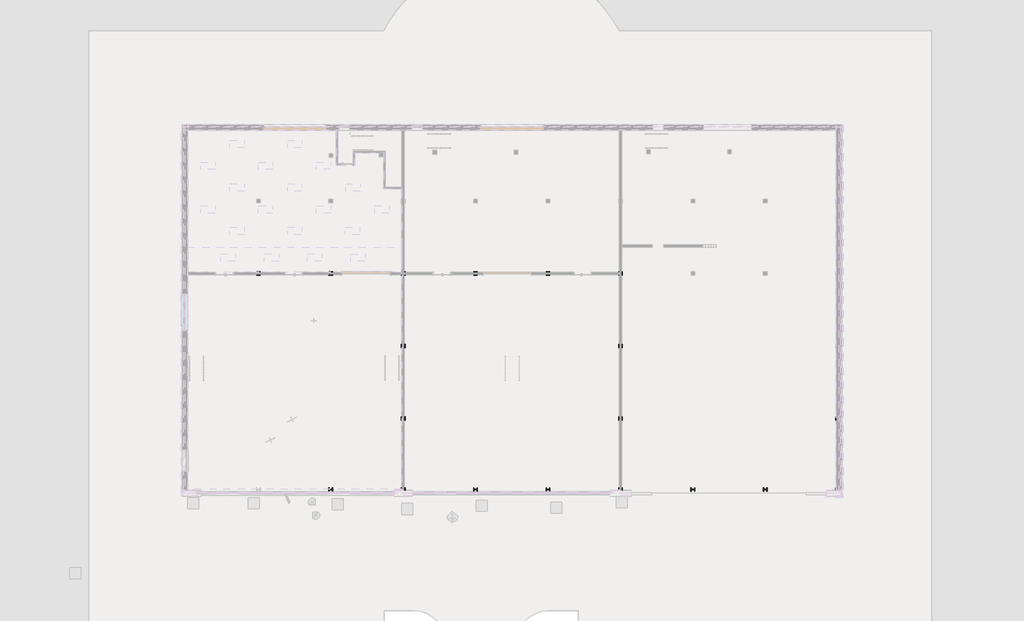
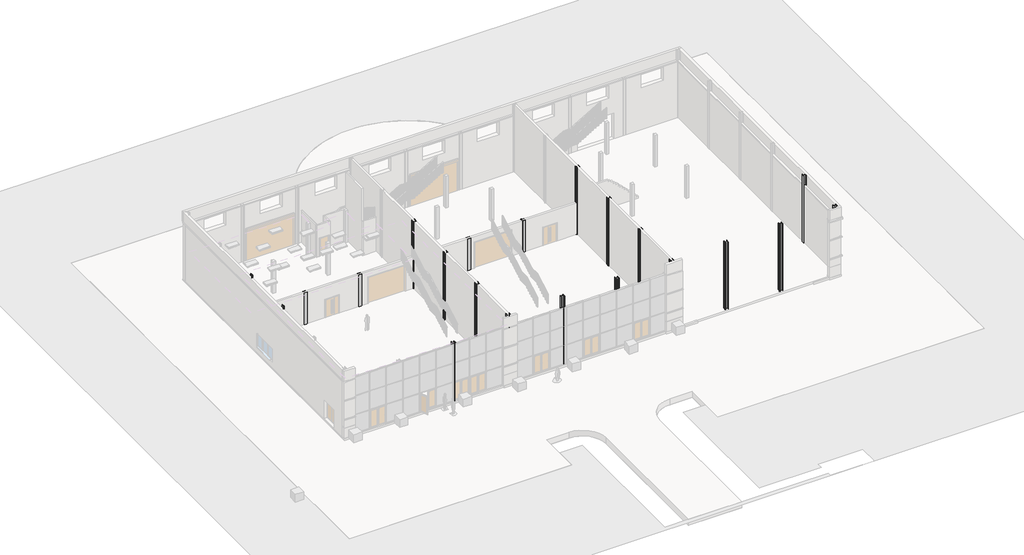
# One storey, part 5 of 13: 21 columns, 21 slabs, 8 footings.
"""IFC4 building model written with IfcOpenShell, lengths in millimetres."""

import ifcopenshell
import ifcopenshell.guid

model = None  # the IFC model being written
_history = None  # IfcOwnerHistory: only IFC2X3 demands one
_inside = {}  # id of a spatial element -> (the spatial element, [elements in it])
_under = {}  # id of a project, library or spatial element -> (it, [spatial elements below it])
_declared = {}  # id of a project -> (the project, [libraries it declares])
_typed = {}  # id of a type object -> (the type object, [elements of that type])
_made_of = {}  # id of a material, layer set ... -> (it, [elements and type objects made of it])


def new_model(schema):
    """Start an empty IFC model of exactly this schema.

    Asked for "IFC4X3", IfcOpenShell would pick the latest addendum, in which some entities
    have other attributes; the version numbers below select the first issue.
    IFC2X3 requires an IfcOwnerHistory on every rooted entity: one is made here for all.
    """
    global model, _history
    if schema == "IFC4X3":
        model = ifcopenshell.file(schema_version=(4, 3, 0, 0))
    else:
        model = ifcopenshell.file(schema=schema)
    _inside.clear()
    _under.clear()
    _declared.clear()
    _typed.clear()
    _made_of.clear()
    _history = None
    if model.schema == "IFC2X3":
        org = make("IfcOrganization", Name="unknown")
        user = make(
            "IfcPersonAndOrganization",
            ThePerson=make("IfcPerson", FamilyName="unknown"),
            TheOrganization=org,
        )
        app = make(
            "IfcApplication",
            ApplicationDeveloper=org,
            Version="unknown",
            ApplicationFullName="unknown",
            ApplicationIdentifier="unknown",
        )
        _history = make(
            "IfcOwnerHistory",
            OwningUser=user,
            OwningApplication=app,
            ChangeAction="ADDED",
            CreationDate=0,
        )
    return model


def make(cls, **values):
    """One entity of the class cls with the attributes given. An attribute that is None is left unset."""
    return model.create_entity(
        cls, **{name: value for name, value in values.items() if value is not None}
    )


def rooted(cls, **values):
    """An entity with a GlobalId (a new one), such as an element, a storey or a relation."""
    return make(cls, GlobalId=ifcopenshell.guid.new(), OwnerHistory=_history, **values)


def si_unit(unit_type, name, prefix=None):
    """IfcSIUnit, for example si_unit("LENGTHUNIT", "METRE", prefix="MILLI")."""
    return make("IfcSIUnit", UnitType=unit_type, Prefix=prefix, Name=name)


def assignment(units):
    """IfcUnitAssignment: the units of a project."""
    return None if units is None else make("IfcUnitAssignment", Units=units)


def point(xyz):
    """IfcCartesianPoint."""
    return None if xyz is None else make("IfcCartesianPoint", Coordinates=xyz)


def direction(xyz):
    """IfcDirection."""
    return None if xyz is None else make("IfcDirection", DirectionRatios=xyz)


def frame(location, z_axis=None, x_axis=None):
    """IfcAxis2Placement3D, a coordinate frame: its origin and axes. An axis left out is left unset."""
    return make(
        "IfcAxis2Placement3D",
        Location=point(location),
        Axis=direction(z_axis),
        RefDirection=direction(x_axis),
    )


def frame_2d(location, x_axis=None):
    """IfcAxis2Placement2D, a coordinate frame in the plane: its origin and x axis."""
    return make(
        "IfcAxis2Placement2D", Location=point(location), RefDirection=direction(x_axis)
    )


def origin():
    """The frame at (0, 0, 0) with its axes left unset."""
    return frame((0.0, 0.0, 0.0))


def place(relative_to, where):
    """IfcLocalPlacement: puts the frame where relative to a parent placement (None: the world)."""
    return make(
        "IfcLocalPlacement", PlacementRelTo=relative_to, RelativePlacement=where
    )


def context(
    kind, dimensions, precision=None, world=None, true_north=None, identifier=None
):
    """IfcGeometricRepresentationContext, for example the 3D "Model" context."""
    return make(
        "IfcGeometricRepresentationContext",
        ContextIdentifier=identifier,
        ContextType=kind,
        CoordinateSpaceDimension=dimensions,
        Precision=precision,
        WorldCoordinateSystem=world,
        TrueNorth=true_north,
    )


def project(units=None, contexts=None):
    """IfcProject with its units and contexts."""
    return rooted(
        "IfcProject",
        Name="project",
        RepresentationContexts=contexts,
        UnitsInContext=assignment(units),
    )


def spatial(cls, under=None, at=None, **own):
    """A site, building, storey or space (cls), placed at a placement, below another one or the project."""
    s = rooted(cls, ObjectPlacement=at, **own)
    if under is not None:
        _under.setdefault(under.id(), (under, []))[1].append(s)
    return s


def polyline(points):
    """IfcPolyline through the points."""
    return make("IfcPolyline", Points=[point(p) for p in points])


def circle_curve(where, radius):
    """IfcCircle in the frame where."""
    return make("IfcCircle", Position=where, Radius=radius)


def trimmed(basis, trim1, trim2, sense, master):
    """IfcTrimmedCurve: the piece of a basis curve between two trims."""
    return make(
        "IfcTrimmedCurve",
        BasisCurve=basis,
        Trim1=trim1,
        Trim2=trim2,
        SenseAgreement=sense,
        MasterRepresentation=master,
    )


def segment(curve, same_sense, transition):
    """IfcCompositeCurveSegment."""
    return make(
        "IfcCompositeCurveSegment",
        Transition=transition,
        SameSense=same_sense,
        ParentCurve=curve,
    )


def composite_curve(segments, self_intersect=None):
    """IfcCompositeCurve: segments joined end to end."""
    return make("IfcCompositeCurve", Segments=segments, SelfIntersect=self_intersect)


def outline(outer, holes=None, kind="AREA"):
    """IfcArbitraryClosedProfileDef: a profile drawn as a closed curve; with holes, ...WithVoids."""
    if holes is None:
        return make("IfcArbitraryClosedProfileDef", ProfileType=kind, OuterCurve=outer)
    return make(
        "IfcArbitraryProfileDefWithVoids",
        ProfileType=kind,
        OuterCurve=outer,
        InnerCurves=holes,
    )


def extrude(swept, where, along, depth):
    """IfcExtrudedAreaSolid: the profile swept, set in the frame where, extruded along a direction by depth."""
    return make(
        "IfcExtrudedAreaSolid",
        SweptArea=swept,
        Position=where,
        ExtrudedDirection=direction(along),
        Depth=depth,
    )


def faces_of(points, faces, orient=None, outer=None):
    """IfcFace entities. A face is a list of loops; a loop is a list of indices into points, from 0.

    orient and outer hold one flag for each loop. By default every Orientation is true, the
    first loop of a face is its IfcFaceOuterBound and the others are IfcFaceBound.
    """
    made = []
    for i, loops in enumerate(faces):
        bounds = []
        for j, loop in enumerate(loops):
            is_outer = j == 0 if outer is None else outer[i][j]
            bounds.append(
                make(
                    "IfcFaceOuterBound" if is_outer else "IfcFaceBound",
                    Bound=make("IfcPolyLoop", Polygon=[points[k] for k in loop]),
                    Orientation=True if orient is None else orient[i][j],
                )
            )
        made.append(make("IfcFace", Bounds=bounds))
    return made


def faceted_brep(points, faces, orient=None, outer=None, voids=None):
    """IfcFacetedBrep: a solid bounded by flat faces; with voids (closed shells), ...WithVoids."""
    shared = [point(p) for p in points]
    hull = make("IfcClosedShell", CfsFaces=faces_of(shared, faces, orient, outer))
    if voids is None:
        return make("IfcFacetedBrep", Outer=hull)
    return make(
        "IfcFacetedBrepWithVoids",
        Outer=hull,
        Voids=[
            make(cls, CfsFaces=faces_of(shared, fs, o, b)) for cls, fs, o, b in voids
        ],
    )


def shape(context_of_items, identifier, shape_type, items):
    """IfcShapeRepresentation: the items that make up one representation, for example the "Body"."""
    return make(
        "IfcShapeRepresentation",
        ContextOfItems=context_of_items,
        RepresentationIdentifier=identifier,
        RepresentationType=shape_type,
        Items=items,
    )


def source(mapping_origin, context_of_items, identifier, shape_type, items):
    """IfcRepresentationMap: a shape defined once, which mapped items show again and again."""
    return make(
        "IfcRepresentationMap",
        MappingOrigin=mapping_origin,
        MappedRepresentation=shape(context_of_items, identifier, shape_type, items),
    )


def transform(
    local_origin,
    x_axis=None,
    y_axis=None,
    z_axis=None,
    scale=None,
    scale2=None,
    scale3=None,
    uniform=True,
):
    """IfcCartesianTransformationOperator3D, or its non-uniform kind. x_axis, y_axis, z_axis: its Axis1, 2, 3."""
    if uniform:
        return make(
            "IfcCartesianTransformationOperator3D",
            Axis1=direction(x_axis),
            Axis2=direction(y_axis),
            LocalOrigin=point(local_origin),
            Scale=scale,
            Axis3=direction(z_axis),
        )
    return make(
        "IfcCartesianTransformationOperator3DnonUniform",
        Axis1=direction(x_axis),
        Axis2=direction(y_axis),
        LocalOrigin=point(local_origin),
        Scale=scale,
        Axis3=direction(z_axis),
        Scale2=scale2,
        Scale3=scale3,
    )


def mapped(mapping_source, mapping_target):
    """IfcMappedItem: shows the shape of a source again, moved by a transform."""
    return make(
        "IfcMappedItem", MappingSource=mapping_source, MappingTarget=mapping_target
    )


def made_of(thing, what):
    """Note that an element or type object is made of a material, layer set ...; save() writes the relation."""
    if what is not None:
        _made_of.setdefault(what.id(), (what, []))[1].append(thing)
    return thing


def element(
    cls,
    number,
    at=None,
    inside=None,
    cuts=None,
    type_object=None,
    material=None,
    context=None,
    identifier="Body",
    shape_type=None,
    held_by="IfcProductDefinitionShape",
    body=None,
    shapes=None,
    **own,
):
    """One element of the class cls, such as IfcWall. Its Tag is "e" and its number.

    at: its placement. inside: the storey or other place that contains it. cuts: it is an
    opening in that element (IfcRelVoidsElement). A single representation is given by context,
    identifier, shape_type and body (its items); several are given by shapes. held_by: the class
    of the entity that holds the representations. save() writes the other relations.
    """
    e = rooted(cls, Tag="e%d" % number, ObjectPlacement=at, **own)
    if body is not None:
        shapes = [shape(context, identifier, shape_type, body)]
    if shapes is not None:
        e.Representation = make(held_by, Representations=shapes)
    if inside is not None:
        _inside.setdefault(inside.id(), (inside, []))[1].append(e)
    if cuts is not None:
        rooted(
            "IfcRelVoidsElement", RelatingBuildingElement=cuts, RelatedOpeningElement=e
        )
    if type_object is not None:
        _typed.setdefault(type_object.id(), (type_object, []))[1].append(e)
    return made_of(e, material)


def aggregate(whole, parts):
    """IfcRelAggregates: a whole, such as a stair, and the parts it consists of."""
    return rooted("IfcRelAggregates", RelatingObject=whole, RelatedObjects=parts)


def save(model, path):
    """Write the relations noted so far, then the file.

    IfcRelAggregates (storeys below a building ...), IfcRelContainedInSpatialStructure (elements
    in a storey), IfcRelDefinesByType, IfcRelAssociatesMaterial and IfcRelDeclares: one each for
    every whole, place, type object, material and project.
    """
    for whole, parts in _under.values():
        aggregate(whole, parts)
    for where, things in _inside.values():
        rooted(
            "IfcRelContainedInSpatialStructure",
            RelatedElements=things,
            RelatingStructure=where,
        )
    for kind, things in _typed.values():
        rooted("IfcRelDefinesByType", RelatedObjects=things, RelatingType=kind)
    for what, things in _made_of.values():
        rooted("IfcRelAssociatesMaterial", RelatedObjects=things, RelatingMaterial=what)
    for by, libraries in _declared.values():
        rooted("IfcRelDeclares", RelatingContext=by, RelatedDefinitions=libraries)
    model.write(path)


def uc_universal_column_column_305x305x97uc_f4bfb62a(model_context):
    return source(origin(), model_context, "Body", "SweptSolid", [
        extrude(outline(composite_curve([segment(polyline([(152.65, 153.95), (152.65, 138.55), (20.15, 138.55)]), True, "CONTINUOUS"), segment(trimmed(circle_curve(frame_2d((20.15, 123.35)), 15.2), [point((20.15, 138.55))], [point((4.95, 123.35))], True, "CARTESIAN"), True, "CONTINUOUS"), segment(polyline([(4.95, 123.35), (4.95, -123.35)]), True, "CONTINUOUS"), segment(trimmed(circle_curve(frame_2d((20.15, -123.35)), 15.2), [point((4.95, -123.35))], [point((20.15, -138.55))], True, "CARTESIAN"), True, "CONTINUOUS"), segment(polyline([(20.15, -138.55), (152.65, -138.55), (152.65, -153.95), (-152.65, -153.95), (-152.65, -138.55), (-20.15, -138.55)]), True, "CONTINUOUS"), segment(trimmed(circle_curve(frame_2d((-20.15, -123.35)), 15.2), [point((-20.15, -138.55))], [point((-4.95, -123.35))], True, "CARTESIAN"), True, "CONTINUOUS"), segment(polyline([(-4.95, -123.35), (-4.95, 123.35)]), True, "CONTINUOUS"), segment(trimmed(circle_curve(frame_2d((-20.15, 123.35)), 15.2), [point((-4.95, 123.35))], [point((-20.15, 138.55))], True, "CARTESIAN"), True, "CONTINUOUS"), segment(polyline([(-20.15, 138.55), (-152.65, 138.55), (-152.65, 153.95), (152.65, 153.95)]), True, "CONTINUOUS")], self_intersect=False)), frame((0.0, 0.0, -1500.0), z_axis=(0.0, 0.0, 1.0), x_axis=(1.0, 0.0, 0.0)), (0.0, 0.0, 1.0), 9300.0),
    ])


def uc_universal_column_column_305x305x97uc_8da79b43(model_context):
    return source(origin(), model_context, "Body", "SweptSolid", [
        extrude(outline(composite_curve([segment(polyline([(152.65, -153.95), (-152.65, -153.95), (-152.65, -138.55), (-20.15, -138.55)]), True, "CONTINUOUS"), segment(trimmed(circle_curve(frame_2d((-20.15, -123.35)), 15.2), [point((-20.15, -138.55))], [point((-4.95, -123.35))], True, "CARTESIAN"), True, "CONTINUOUS"), segment(polyline([(-4.95, -123.35), (-4.95, 123.35)]), True, "CONTINUOUS"), segment(trimmed(circle_curve(frame_2d((-20.15, 123.35)), 15.2), [point((-4.95, 123.35))], [point((-20.15, 138.55))], True, "CARTESIAN"), True, "CONTINUOUS"), segment(polyline([(-20.15, 138.55), (-152.65, 138.55), (-152.65, 153.95), (152.65, 153.95), (152.65, 138.55), (20.15, 138.55)]), True, "CONTINUOUS"), segment(trimmed(circle_curve(frame_2d((20.15, 123.35)), 15.2), [point((20.15, 138.55))], [point((4.95, 123.35))], True, "CARTESIAN"), True, "CONTINUOUS"), segment(polyline([(4.95, 123.35), (4.95, -123.35)]), True, "CONTINUOUS"), segment(trimmed(circle_curve(frame_2d((20.15, -123.35)), 15.2), [point((4.95, -123.35))], [point((20.15, -138.55))], True, "CARTESIAN"), True, "CONTINUOUS"), segment(polyline([(20.15, -138.55), (152.65, -138.55), (152.65, -153.95)]), True, "CONTINUOUS")], self_intersect=False)), frame((0.0, 0.0, -1500.0), z_axis=(0.0, 0.0, 1.0), x_axis=(1.0, 0.0, 0.0)), (0.0, 0.0, 1.0), 9300.0),
    ])


def uc_universal_column_column_305x305x97uc_43a052ce(model_context):
    return source(origin(), model_context, "Body", "SweptSolid", [
        extrude(outline(composite_curve([segment(polyline([(152.65, 153.95), (152.65, 138.55), (20.15, 138.55)]), True, "CONTINUOUS"), segment(trimmed(circle_curve(frame_2d((20.15, 123.35)), 15.2), [point((20.15, 138.55))], [point((4.95, 123.35))], True, "CARTESIAN"), True, "CONTINUOUS"), segment(polyline([(4.95, 123.35), (4.95, -123.35)]), True, "CONTINUOUS"), segment(trimmed(circle_curve(frame_2d((20.15, -123.35)), 15.2), [point((4.95, -123.35))], [point((20.15, -138.55))], True, "CARTESIAN"), True, "CONTINUOUS"), segment(polyline([(20.15, -138.55), (152.65, -138.55), (152.65, -153.95), (-152.65, -153.95), (-152.65, -138.55), (-20.15, -138.55)]), True, "CONTINUOUS"), segment(trimmed(circle_curve(frame_2d((-20.15, -123.35)), 15.2), [point((-20.15, -138.55))], [point((-4.95, -123.35))], True, "CARTESIAN"), True, "CONTINUOUS"), segment(polyline([(-4.95, -123.35), (-4.95, 123.35)]), True, "CONTINUOUS"), segment(trimmed(circle_curve(frame_2d((-20.15, 123.35)), 15.2), [point((-4.95, 123.35))], [point((-20.15, 138.55))], True, "CARTESIAN"), True, "CONTINUOUS"), segment(polyline([(-20.15, 138.55), (-152.65, 138.55), (-152.65, 153.95), (152.65, 153.95)]), True, "CONTINUOUS")], self_intersect=False)), frame((0.0, 0.0, -1500.0), z_axis=(0.0, 0.0, 1.0), x_axis=(1.0, 0.0, 0.0)), (0.0, 0.0, 1.0), 8100.0),
    ])


def pad_foundation_rectangular_1000x1000x500_ed6229e9(model_context):
    return source(origin(), model_context, "Body", "SweptSolid", [
        extrude(outline(polyline([(500.0, 500.0), (500.0, -500.0), (-500.0, -500.0), (-500.0, 500.0), (500.0, 500.0)])), frame((0.0, 0.0, -500.0), z_axis=(0.0, 0.0, 1.0), x_axis=(1.0, 0.0, 0.0)), (0.0, 0.0, 1.0), 500.0),
    ])


model = new_model("IFC4")

# Units and contexts
model_context = context("Model", 3, world=origin())
ifc_project = project(units=[si_unit("LENGTHUNIT", "METRE", prefix="MILLI")], contexts=[model_context])

# Site, building, storey
site = spatial("IfcSite", under=ifc_project)
building = spatial("IfcBuilding", under=site)
storey = spatial("IfcBuildingStorey", under=building, Name="L0 - Ground Floor (Shadows On)", Elevation=0.0)

# Columns
placement = place(None, origin())
element("IfcColumn", 1, ObjectType="Concrete Square : 300 x 300mm", at=placement, inside=storey, context=model_context, shape_type="SweptSolid", body=[
    extrude(outline(polyline([(-989.5553457, -5208.7619082), (-1289.5553457, -5208.7619082), (-1289.5553457, -4908.7619082), (-989.5553457, -4908.7619082), (-989.5553457, -5208.7619082)])), frame((0.0, 0.0, -1500.0), z_axis=(0.0, 0.0, 1.0), x_axis=(1.0, 0.0, 0.0)), (0.0, 0.0, 1.0), 5200.0),
])
element("IfcColumn", 2, ObjectType="Concrete Square : 300 x 300mm", at=placement, inside=storey, context=model_context, shape_type="SweptSolid", body=[
    extrude(outline(polyline([(5010.4446543, -5208.7619082), (4710.4446543, -5208.7619082), (4710.4446543, -4908.7619082), (5010.4446543, -4908.7619082), (5010.4446543, -5208.7619082)])), frame((0.0, 0.0, -1500.0), z_axis=(0.0, 0.0, 1.0), x_axis=(1.0, 0.0, 0.0)), (0.0, 0.0, 1.0), 5200.0),
])
element("IfcColumn", 3, ObjectType="Concrete Square : 300 x 300mm", at=placement, inside=storey, context=model_context, shape_type="SweptSolid", body=[
    extrude(outline(polyline([(17010.4446543, -5208.7619082), (16710.4446543, -5208.7619082), (16710.4446543, -4908.7619082), (17010.4446543, -4908.7619082), (17010.4446543, -5208.7619082)])), frame((0.0, 0.0, -1500.0), z_axis=(0.0, 0.0, 1.0), x_axis=(1.0, 0.0, 0.0)), (0.0, 0.0, 1.0), 5200.0),
])
element("IfcColumn", 4, ObjectType="Concrete Square : 300 x 300mm", at=placement, inside=storey, context=model_context, shape_type="SweptSolid", body=[
    extrude(outline(polyline([(23010.4446543, -5208.7619082), (22710.4446543, -5208.7619082), (22710.4446543, -4908.7619082), (23010.4446543, -4908.7619082), (23010.4446543, -5208.7619082)])), frame((0.0, 0.0, -1500.0), z_axis=(0.0, 0.0, 1.0), x_axis=(1.0, 0.0, 0.0)), (0.0, 0.0, 1.0), 5200.0),
])
element("IfcColumn", 5, ObjectType="UC-Universal Column-Column : 305x305x97UC", at=placement, inside=storey, context=model_context, shape_type="SweptSolid", body=[
    extrude(outline(composite_curve([segment(polyline([(-7293.5053457, -10906.1119082), (-7278.1053457, -10906.1119082), (-7278.1053457, -11038.6119082)]), True, "CONTINUOUS"), segment(trimmed(circle_curve(frame_2d((-7262.9053457, -11038.6119082)), 15.2), [point((-7278.1053457, -11038.6119082))], [point((-7262.9053457, -11053.8119082))], True, "CARTESIAN"), True, "CONTINUOUS"), segment(polyline([(-7262.9053457, -11053.8119082), (-7016.2053457, -11053.8119082)]), True, "CONTINUOUS"), segment(trimmed(circle_curve(frame_2d((-7016.2053457, -11038.6119082)), 15.2), [point((-7016.2053457, -11053.8119082))], [point((-7001.0053457, -11038.6119082))], True, "CARTESIAN"), True, "CONTINUOUS"), segment(polyline([(-7001.0053457, -11038.6119082), (-7001.0053457, -10906.1119082), (-6985.6053457, -10906.1119082), (-6985.6053457, -11211.4119082), (-7001.0053457, -11211.4119082), (-7001.0053457, -11078.9119082)]), True, "CONTINUOUS"), segment(trimmed(circle_curve(frame_2d((-7016.2053457, -11078.9119082)), 15.2), [point((-7001.0053457, -11078.9119082))], [point((-7016.2053457, -11063.7119082))], True, "CARTESIAN"), True, "CONTINUOUS"), segment(polyline([(-7016.2053457, -11063.7119082), (-7262.9053457, -11063.7119082)]), True, "CONTINUOUS"), segment(trimmed(circle_curve(frame_2d((-7262.9053457, -11078.9119082)), 15.2), [point((-7262.9053457, -11063.7119082))], [point((-7278.1053457, -11078.9119082))], True, "CARTESIAN"), True, "CONTINUOUS"), segment(polyline([(-7278.1053457, -11078.9119082), (-7278.1053457, -11211.4119082), (-7293.5053457, -11211.4119082), (-7293.5053457, -10906.1119082)]), True, "CONTINUOUS")], self_intersect=False)), frame((0.0, 0.0, -1500.0), z_axis=(0.0, 0.0, 1.0), x_axis=(1.0, 0.0, 0.0)), (0.0, 0.0, 1.0), 9300.0),
])
element("IfcColumn", 6, ObjectType="UC-Universal Column-Column : 305x305x97UC", at=placement, inside=storey, context=model_context, shape_type="SweptSolid", body=[
    extrude(outline(composite_curve([segment(polyline([(-7293.5053457, -4906.1119082), (-7278.1053457, -4906.1119082), (-7278.1053457, -5038.6119082)]), True, "CONTINUOUS"), segment(trimmed(circle_curve(frame_2d((-7262.9053457, -5038.6119082)), 15.2), [point((-7278.1053457, -5038.6119082))], [point((-7262.9053457, -5053.8119082))], True, "CARTESIAN"), True, "CONTINUOUS"), segment(polyline([(-7262.9053457, -5053.8119082), (-7016.2053457, -5053.8119082)]), True, "CONTINUOUS"), segment(trimmed(circle_curve(frame_2d((-7016.2053457, -5038.6119082)), 15.2), [point((-7016.2053457, -5053.8119082))], [point((-7001.0053457, -5038.6119082))], True, "CARTESIAN"), True, "CONTINUOUS"), segment(polyline([(-7001.0053457, -5038.6119082), (-7001.0053457, -4906.1119082), (-6985.6053457, -4906.1119082), (-6985.6053457, -5211.4119082), (-7001.0053457, -5211.4119082), (-7001.0053457, -5078.9119082)]), True, "CONTINUOUS"), segment(trimmed(circle_curve(frame_2d((-7016.2053457, -5078.9119082)), 15.2), [point((-7001.0053457, -5078.9119082))], [point((-7016.2053457, -5063.7119082))], True, "CARTESIAN"), True, "CONTINUOUS"), segment(polyline([(-7016.2053457, -5063.7119082), (-7262.9053457, -5063.7119082)]), True, "CONTINUOUS"), segment(trimmed(circle_curve(frame_2d((-7262.9053457, -5078.9119082)), 15.2), [point((-7262.9053457, -5063.7119082))], [point((-7278.1053457, -5078.9119082))], True, "CARTESIAN"), True, "CONTINUOUS"), segment(polyline([(-7278.1053457, -5078.9119082), (-7278.1053457, -5211.4119082), (-7293.5053457, -5211.4119082), (-7293.5053457, -4906.1119082)]), True, "CONTINUOUS")], self_intersect=False)), frame((0.0, 0.0, -1500.0), z_axis=(0.0, 0.0, 1.0), x_axis=(1.0, 0.0, 0.0)), (0.0, 0.0, 1.0), 9300.0),
])
uc_universal_column_column_305x305x97uc_shape = uc_universal_column_column_305x305x97uc_f4bfb62a(model_context)
element("IfcColumn", 7, ObjectType="UC-Universal Column-Column : 305x305x97UC", at=placement, inside=storey, context=model_context, shape_type="MappedRepresentation", body=[
    mapped(uc_universal_column_column_305x305x97uc_shape, transform((10860.4446543, -17058.7619082, 0.0), x_axis=(0.0, 1.0, 0.0), y_axis=(-1.0, 0.0, 0.0), z_axis=(0.0, 0.0, 1.0))),
])
element("IfcColumn", 8, ObjectType="UC-Universal Column-Column : 305x305x97UC", at=placement, inside=storey, context=model_context, shape_type="MappedRepresentation", body=[
    mapped(uc_universal_column_column_305x305x97uc_shape, transform((28860.4446543, -17058.7619082, 0.0), x_axis=(0.0, 1.0, 0.0), y_axis=(-1.0, 0.0, 0.0), z_axis=(0.0, 0.0, 1.0))),
])
element("IfcColumn", 9, ObjectType="UC-Universal Column-Column : 305x305x97UC", at=placement, inside=storey, context=model_context, shape_type="MappedRepresentation", body=[
    mapped(uc_universal_column_column_305x305x97uc_shape, transform((10860.4446543, -11058.7619082, 0.0), x_axis=(0.0, 1.0, 0.0), y_axis=(-1.0, 0.0, 0.0), z_axis=(0.0, 0.0, 1.0))),
])
element("IfcColumn", 10, ObjectType="UC-Universal Column-Column : 305x305x97UC", at=placement, inside=storey, context=model_context, shape_type="MappedRepresentation", body=[
    mapped(uc_universal_column_column_305x305x97uc_shape, transform((28860.4446543, -11058.7619082, 0.0), x_axis=(0.0, 1.0, 0.0), y_axis=(-1.0, 0.0, 0.0), z_axis=(0.0, 0.0, 1.0))),
])
element("IfcColumn", 11, ObjectType="UC-Universal Column-Column : 305x305x97UC", at=placement, inside=storey, context=model_context, shape_type="MappedRepresentation", body=[
    mapped(uc_universal_column_column_305x305x97uc_shape, transform((10860.4446543, -5058.7619082, 0.0), x_axis=(0.0, 1.0, 0.0), y_axis=(-1.0, 0.0, 0.0), z_axis=(0.0, 0.0, 1.0))),
])
element("IfcColumn", 12, ObjectType="UC-Universal Column-Column : 305x305x97UC", at=placement, inside=storey, context=model_context, shape_type="MappedRepresentation", body=[
    mapped(uc_universal_column_column_305x305x97uc_shape, transform((28860.4446543, -5058.7619082, 0.0), x_axis=(0.0, 1.0, 0.0), y_axis=(-1.0, 0.0, 0.0), z_axis=(0.0, 0.0, 1.0))),
])
element("IfcColumn", 13, ObjectType="UC-Universal Column-Column : 305x305x97UC", at=placement, inside=storey, context=model_context, shape_type="MappedRepresentation", body=[
    mapped(uc_universal_column_column_305x305x97uc_shape, transform((10860.4446543, -22948.7619082, 0.0), x_axis=(0.0, 1.0, 0.0), y_axis=(-1.0, 0.0, 0.0), z_axis=(0.0, 0.0, 1.0))),
])
element("IfcColumn", 14, ObjectType="UC-Universal Column-Column : 305x305x97UC", at=placement, inside=storey, context=model_context, shape_type="MappedRepresentation", body=[
    mapped(uc_universal_column_column_305x305x97uc_shape, transform((16860.4446543, -22948.7619082, 0.0), x_axis=(0.0, 1.0, 0.0), y_axis=(-1.0, 0.0, 0.0), z_axis=(0.0, 0.0, 1.0))),
])
element("IfcColumn", 15, ObjectType="UC-Universal Column-Column : 305x305x97UC", at=placement, inside=storey, context=model_context, shape_type="MappedRepresentation", body=[
    mapped(uc_universal_column_column_305x305x97uc_shape, transform((22860.4446543, -22948.7619082, 0.0), x_axis=(0.0, 1.0, 0.0), y_axis=(-1.0, 0.0, 0.0), z_axis=(0.0, 0.0, 1.0))),
])
element("IfcColumn", 16, ObjectType="UC-Universal Column-Column : 305x305x97UC", at=placement, inside=storey, context=model_context, shape_type="MappedRepresentation", body=[
    mapped(uc_universal_column_column_305x305x97uc_shape, transform((34860.4446543, -22948.7619082, 0.0), x_axis=(0.0, 1.0, 0.0), y_axis=(-1.0, 0.0, 0.0), z_axis=(0.0, 0.0, 1.0))),
])
element("IfcColumn", 17, ObjectType="UC-Universal Column-Column : 305x305x97UC", at=placement, inside=storey, context=model_context, shape_type="MappedRepresentation", body=[
    mapped(uc_universal_column_column_305x305x97uc_shape, transform((28860.4446543, -22948.7619082, 0.0), x_axis=(0.0, 1.0, 0.0), y_axis=(-1.0, 0.0, 0.0), z_axis=(0.0, 0.0, 1.0))),
])
element("IfcColumn", 18, ObjectType="UC-Universal Column-Column : 305x305x97UC", at=placement, inside=storey, context=model_context, shape_type="MappedRepresentation", body=[
    mapped(uc_universal_column_column_305x305x97uc_shape, transform((40860.4446543, -22948.7619082, 0.0), x_axis=(0.0, 1.0, 0.0), y_axis=(-1.0, 0.0, 0.0), z_axis=(0.0, 0.0, 1.0))),
])
uc_universal_column_column_305x305x97uc_2_shape = uc_universal_column_column_305x305x97uc_8da79b43(model_context)
element("IfcColumn", 19, ObjectType="UC-Universal Column-Column : 305x305x97UC", at=placement, inside=storey, context=model_context, shape_type="MappedRepresentation", body=[
    mapped(uc_universal_column_column_305x305x97uc_2_shape, transform((46860.4446543, -22948.7619082, 0.0), x_axis=(0.0, 1.0, 0.0), y_axis=(-1.0, 0.0, 0.0), z_axis=(0.0, 0.0, 1.0))),
])
element("IfcColumn", 20, ObjectType="UC-Universal Column-Column : 305x305x97UC", at=placement, inside=storey, context=model_context, shape_type="MappedRepresentation", body=[
    mapped(uc_universal_column_column_305x305x97uc_2_shape, transform((46860.4446543, -17058.7619082, 0.0), x_axis=(0.0, 1.0, 0.0), y_axis=(-1.0, 0.0, 0.0), z_axis=(0.0, 0.0, 1.0))),
])
uc_universal_column_column_305x305x97uc_3_shape = uc_universal_column_column_305x305x97uc_43a052ce(model_context)
element("IfcColumn", 21, ObjectType="UC-Universal Column-Column : 305x305x97UC", at=placement, inside=storey, context=model_context, shape_type="MappedRepresentation", body=[
    mapped(uc_universal_column_column_305x305x97uc_3_shape, transform((4860.4446543, -22948.7619082, 0.0), x_axis=(0.0, 1.0, 0.0), y_axis=(-1.0, 0.0, 0.0), z_axis=(0.0, 0.0, 1.0))),
])

# Footings
element("IfcFooting", 22, ObjectType="Wall Foundation - Commercial 1300 x 450", at=placement, inside=storey, context=model_context, shape_type="Brep", body=[
    faceted_brep([(-7673.2053457, 7505.9380918, -1200.0), (-7673.2053457, -23738.4619082, -1200.0), (-6758.8053457, -23738.4619082, -1200.0), (-6758.8053457, -22824.0619082, -1200.0), (-6758.8053457, 6591.5380918, -1200.0), (-6758.8053457, 7505.9380918, -1200.0), (-7673.2053457, 7505.9380918, -1504.8), (-7673.2053457, -23738.4619082, -1504.8), (-6758.8053457, 7505.9380918, -1504.8), (-6758.8053457, 7441.2380918, -1504.8), (-7639.5553457, 7441.2380918, -1504.8), (-7639.5553457, 6441.2380918, -1504.8), (-6758.8053457, 6441.2380918, -1504.8), (-6758.8053457, 1441.2380918, -1504.8), (-7639.5553457, 1441.2380918, -1504.8), (-7639.5553457, 441.2380918, -1504.8), (-6758.8053457, 441.2380918, -1504.8), (-6758.8053457, -4558.7619082, -1504.8), (-7639.5553457, -4558.7619082, -1504.8), (-7639.5553457, -5558.7619082, -1504.8), (-6758.8053457, -5558.7619082, -1504.8), (-6758.8053457, -10558.7619082, -1504.8), (-7639.5553457, -10558.7619082, -1504.8), (-7639.5553457, -11558.7619082, -1504.8), (-6758.8053457, -11558.7619082, -1504.8), (-6758.8053457, -16558.7619082, -1504.8), (-7639.5553457, -16558.7619082, -1504.8), (-7639.5553457, -17558.7619082, -1504.8), (-6758.8053457, -17558.7619082, -1504.8), (-6758.8053457, -22448.7619082, -1504.8), (-7639.5553457, -22448.7619082, -1504.8), (-7639.5553457, -23448.7619082, -1504.8), (-6758.8053457, -23448.7619082, -1504.8), (-6758.8053457, -23738.4619082, -1504.8), (-6758.8053457, -23448.7619082, -1500.0), (-6758.8053457, -22824.0619082, -1500.0), (-6758.8053457, -22448.7619082, -1500.0), (-6758.8053457, -17558.7619082, -1500.0), (-6758.8053457, -16558.7619082, -1500.0), (-6758.8053457, -11558.7619082, -1500.0), (-6758.8053457, -10558.7619082, -1500.0), (-6758.8053457, -5558.7619082, -1500.0), (-6758.8053457, -4558.7619082, -1500.0), (-6758.8053457, 441.2380918, -1500.0), (-6758.8053457, 1441.2380918, -1500.0), (-6758.8053457, 6441.2380918, -1500.0), (-6758.8053457, 6591.5380918, -1500.0), (-6758.8053457, 7441.2380918, -1500.0), (-7639.5553457, 441.2380918, -1500.0), (-7639.5553457, 1441.2380918, -1500.0), (-7639.5553457, 6441.2380918, -1500.0), (-7639.5553457, 7441.2380918, -1500.0), (-7639.5553457, -5558.7619082, -1500.0), (-7639.5553457, -4558.7619082, -1500.0), (-7639.5553457, -11558.7619082, -1500.0), (-7639.5553457, -10558.7619082, -1500.0), (-7639.5553457, -17558.7619082, -1500.0), (-7639.5553457, -16558.7619082, -1500.0), (-7639.5553457, -23448.7619082, -1500.0), (-7639.5553457, -22448.7619082, -1500.0)], [[[0, 1, 2, 3, 4, 5]], [[1, 0, 6, 7]], [[7, 6, 8, 9, 10, 11, 12, 13, 14, 15, 16, 17, 18, 19, 20, 21, 22, 23, 24, 25, 26, 27, 28, 29, 30, 31, 32, 33]], [[5, 4, 3, 2, 33, 32, 34, 35, 36, 29, 28, 37, 38, 25, 24, 39, 40, 21, 20, 41, 42, 17, 16, 43, 44, 13, 12, 45, 46, 47, 9, 8]], [[2, 1, 7, 33]], [[48, 49, 44, 43]], [[44, 49, 14, 13]], [[49, 48, 15, 14]], [[48, 43, 16, 15]], [[50, 51, 47, 46, 45]], [[51, 50, 11, 10]], [[50, 45, 12, 11]], [[52, 53, 42, 41]], [[42, 53, 18, 17]], [[53, 52, 19, 18]], [[52, 41, 20, 19]], [[54, 55, 40, 39]], [[40, 55, 22, 21]], [[55, 54, 23, 22]], [[54, 39, 24, 23]], [[56, 57, 38, 37]], [[38, 57, 26, 25]], [[57, 56, 27, 26]], [[56, 37, 28, 27]], [[58, 59, 36, 35, 34]], [[36, 59, 30, 29]], [[59, 58, 31, 30]], [[0, 5, 8, 6]], [[47, 51, 10, 9]], [[58, 34, 32, 31]]]),
])
element("IfcFooting", 23, ObjectType="Wall Foundation - Commercial 1300 x 450", at=placement, inside=storey, context=model_context, shape_type="Brep", body=[
    faceted_brep([(11600.0976476, -23733.4474846, -1200.0), (11600.0976476, -23733.4474846, -1504.8), (11600.0976476, -23618.4474846, -1504.8), (11600.0976476, -22819.0474846, -1504.8), (11600.0976476, -22819.0474846, -1200.0), (11600.0976476, -23618.4474846, -1200.0), (10120.0976476, -23733.4474846, -1504.8), (10120.0976476, -23733.4474846, -1200.0), (10120.0976476, -23625.2469755, -1200.0), (10120.0976476, -22819.0474846, -1200.0), (10120.0976476, -22819.0474846, -1504.8), (10120.0976476, -23625.2469755, -1504.8), (11317.6446543, -22819.0474846, -1200.0), (10403.2446543, -22819.0474846, -1200.0), (10360.4446543, -22819.0474846, -1504.8), (10360.4446543, -23448.7619082, -1504.8), (11360.4446543, -23448.7619082, -1504.8), (11360.4446543, -22819.0474846, -1504.8), (11360.4446543, -22819.0474846, -1500.0), (11317.6446543, -22819.0474846, -1500.0), (10403.2446543, -22819.0474846, -1500.0), (10360.4446543, -22819.0474846, -1500.0), (11360.4446543, -23448.7619082, -1500.0), (10360.4446543, -23448.7619082, -1500.0)], [[[0, 1, 2, 3, 4, 5]], [[6, 7, 8, 9, 10, 11]], [[7, 0, 5, 4, 12, 13, 9, 8]], [[1, 0, 7, 6]], [[3, 2, 1, 6, 11, 10, 14, 15, 16, 17]], [[4, 3, 17, 18, 19, 20, 21, 14, 10, 9, 13, 12]], [[22, 23, 21, 20, 19, 18]], [[21, 23, 15, 14]], [[23, 22, 16, 15]], [[22, 18, 17, 16]]]),
])
element("IfcFooting", 24, ObjectType="Wall Foundation - Commercial 1300 x 450", at=placement, inside=storey, context=model_context, shape_type="Brep", body=[
    faceted_brep([(31560.0976476, -23733.4474846, -1200.0), (31560.0976476, -23733.4474846, -1504.8), (31560.0976476, -22819.0474846, -1504.8), (31560.0976476, -22819.0474846, -1200.0), (27960.0976476, -23733.4474846, -1504.8), (27960.0976476, -23733.4474846, -1200.0), (27960.0976476, -23618.4474846, -1200.0), (27960.0976476, -22819.0474846, -1200.0), (27960.0976476, -22819.0474846, -1504.8), (27960.0976476, -23618.4474846, -1504.8), (29317.6446543, -22819.0474846, -1200.0), (28403.2446543, -22819.0474846, -1200.0), (28360.4446543, -22819.0474846, -1504.8), (28360.4446543, -23448.7619082, -1504.8), (29360.4446543, -23448.7619082, -1504.8), (29360.4446543, -22819.0474846, -1504.8), (29360.4446543, -22819.0474846, -1500.0), (29317.6446543, -22819.0474846, -1500.0), (28403.2446543, -22819.0474846, -1500.0), (28360.4446543, -22819.0474846, -1500.0), (29360.4446543, -23448.7619082, -1500.0), (28360.4446543, -23448.7619082, -1500.0)], [[[0, 1, 2, 3]], [[4, 5, 6, 7, 8, 9]], [[5, 0, 3, 10, 11, 7, 6]], [[1, 0, 5, 4]], [[2, 1, 4, 9, 8, 12, 13, 14, 15]], [[3, 2, 15, 16, 17, 18, 19, 12, 8, 7, 11, 10]], [[20, 21, 19, 18, 17, 16]], [[19, 21, 13, 12]], [[21, 20, 14, 13]], [[20, 16, 15, 14]]]),
])
element("IfcFooting", 25, ObjectType="Wall Foundation - Commercial 1300 x 450", at=placement, inside=storey, context=model_context, shape_type="Brep", body=[
    faceted_brep([(43960.0976476, -23733.4474846, -1504.8), (43960.0976476, -23733.4474846, -1200.0), (43960.0976476, -22819.0474846, -1200.0), (43960.0976476, -22819.0474846, -1504.8), (47425.1446543, -23733.4474846, -1200.0), (47425.1446543, -22819.0474846, -1200.0), (46510.7446543, -22819.0474846, -1200.0), (47425.1446543, -23733.4474846, -1504.8), (46360.4446543, -22819.0474846, -1504.8), (46360.4446543, -23448.7619082, -1504.8), (47360.4446543, -23448.7619082, -1504.8), (47360.4446543, -22819.0474846, -1504.8), (47425.1446543, -22819.0474846, -1504.8), (47360.4446543, -22819.0474846, -1500.0), (46510.7446543, -22819.0474846, -1500.0), (46360.4446543, -22819.0474846, -1500.0), (47360.4446543, -23448.7619082, -1500.0), (46360.4446543, -23448.7619082, -1500.0)], [[[0, 1, 2, 3]], [[1, 4, 5, 6, 2]], [[1, 0, 7, 4]], [[0, 3, 8, 9, 10, 11, 12, 7]], [[3, 2, 6, 5, 12, 11, 13, 14, 15, 8]], [[16, 17, 15, 14, 13]], [[15, 17, 9, 8]], [[17, 16, 10, 9]], [[5, 4, 7, 12]], [[16, 13, 11, 10]]]),
])
element("IfcFooting", 26, ObjectType="Wall Foundation - Commercial 1300 x 450", at=placement, inside=storey, context=model_context, shape_type="SweptSolid", body=[
    extrude(outline(polyline([(1441.2380918, -1500.0), (441.2380918, -1500.0), (441.2380918, -1504.8), (-4558.7619082, -1504.8), (-4558.7619082, -1500.0), (-5558.7619082, -1500.0), (-5558.7619082, -1504.8), (-10558.7619082, -1504.8), (-10558.7619082, -1500.0), (-11558.7619082, -1500.0), (-11558.7619082, -1504.8), (-16558.7619082, -1504.8), (-16558.7619082, -1500.0), (-17558.7619082, -1500.0), (-17558.7619082, -1504.8), (-22448.7619082, -1504.8), (-22448.7619082, -1500.0), (-22819.0474846, -1500.0), (-22819.0474846, -1200.0), (6591.5380918, -1200.0), (6591.5380918, -1500.0), (6441.2380918, -1500.0), (6441.2380918, -1504.8), (1441.2380918, -1504.8), (1441.2380918, -1500.0)])), frame((28403.2446543, 0.0, 0.0), z_axis=(1.0, 0.0, 0.0), x_axis=(0.0, 1.0, 0.0)), (0.0, 0.0, 1.0), 914.4),
])
element("IfcFooting", 27, ObjectType="Wall Foundation - Commercial 1300 x 450", at=placement, inside=storey, context=model_context, shape_type="SweptSolid", body=[
    extrude(outline(polyline([(1441.2380918, -1500.0), (441.2380918, -1500.0), (441.2380918, -1504.8), (-4558.7619082, -1504.8), (-4558.7619082, -1500.0), (-5558.7619082, -1500.0), (-5558.7619082, -1504.8), (-10558.7619082, -1504.8), (-10558.7619082, -1500.0), (-11558.7619082, -1500.0), (-11558.7619082, -1504.8), (-16558.7619082, -1504.8), (-16558.7619082, -1500.0), (-17558.7619082, -1500.0), (-17558.7619082, -1504.8), (-22448.7619082, -1504.8), (-22448.7619082, -1500.0), (-22819.0474846, -1500.0), (-22819.0474846, -1200.0), (6591.5380918, -1200.0), (6591.5380918, -1500.0), (6441.2380918, -1500.0), (6441.2380918, -1504.8), (1441.2380918, -1504.8), (1441.2380918, -1500.0)])), frame((10403.2446543, 0.0, 0.0), z_axis=(1.0, 0.0, 0.0), x_axis=(0.0, 1.0, 0.0)), (0.0, 0.0, 1.0), 914.4),
])
element("IfcFooting", 28, ObjectType="Wall Foundation - Commercial 1300 x 450", at=placement, inside=storey, context=model_context, shape_type="Brep", body=[
    faceted_brep([(-6531.0053457, -22710.8469755, -1200.0), (-6531.0053457, -22710.8469755, -1504.8), (-6531.0053457, -22824.0619082, -1504.8), (-6531.0053457, -23625.2469755, -1504.8), (-6531.0053457, -23625.2469755, -1200.0), (-6531.0053457, -22824.0619082, -1200.0), (10120.0976476, -22710.8469755, -1504.8), (10120.0976476, -22710.8469755, -1200.0), (10120.0976476, -22819.0474846, -1200.0), (10120.0976476, -23625.2469755, -1200.0), (10120.0976476, -23625.2469755, -1504.8), (10120.0976476, -22819.0474846, -1504.8), (-6239.5553457, -23625.2469755, -1200.0), (-6214.1553457, -23625.2469755, -1200.0), (-6214.1553457, -22824.0619082, -1200.0), (-5856.0053457, -22824.0619082, -1200.0), (-5856.0053457, -23625.2469755, -1200.0), (5360.4446543, -22710.8469755, -1504.8), (5360.4446543, -22710.8469755, -1500.0), (4360.4446543, -22710.8469755, -1500.0), (4360.4446543, -22710.8469755, -1504.8), (-639.5553457, -22710.8469755, -1504.8), (-639.5553457, -22710.8469755, -1500.0), (-1639.5553457, -22710.8469755, -1500.0), (-1639.5553457, -22710.8469755, -1504.8), (-1639.5553457, -23448.7619082, -1504.8), (-639.5553457, -23448.7619082, -1504.8), (4360.4446543, -23448.7619082, -1504.8), (5360.4446543, -23448.7619082, -1504.8), (-5856.0053457, -23625.2469755, -1504.8), (-5856.0053457, -22824.0619082, -1504.8), (-6214.1553457, -22824.0619082, -1504.8), (-6214.1553457, -23625.2469755, -1504.8), (-6239.5553457, -23625.2469755, -1504.8), (5360.4446543, -23448.7619082, -1500.0), (4360.4446543, -23448.7619082, -1500.0), (-639.5553457, -23448.7619082, -1500.0), (-1639.5553457, -23448.7619082, -1500.0)], [[[0, 1, 2, 3, 4, 5]], [[6, 7, 8, 9, 10, 11]], [[7, 0, 5, 4, 12, 13, 14, 15, 16, 9, 8]], [[1, 0, 7, 6, 17, 18, 19, 20, 21, 22, 23, 24]], [[3, 2, 1, 24, 25, 26, 21, 20, 27, 28, 17, 6, 11, 10, 29, 30, 31, 32, 33]], [[10, 9, 16, 29]], [[4, 3, 33, 32, 13, 12]], [[34, 35, 19, 18]], [[19, 35, 27, 20]], [[35, 34, 28, 27]], [[34, 18, 17, 28]], [[36, 37, 23, 22]], [[23, 37, 25, 24]], [[37, 36, 26, 25]], [[36, 22, 21, 26]], [[15, 30, 29, 16]], [[30, 15, 14, 31]], [[31, 14, 13, 32]]]),
])
element("IfcFooting", 29, ObjectType="Wall Foundation - Commercial 1300 x 450", at=placement, inside=storey, context=model_context, shape_type="Brep", body=[
    faceted_brep([(27960.0976476, -23618.4474846, -1200.0), (27960.0976476, -23618.4474846, -1504.8), (27960.0976476, -22819.0474846, -1504.8), (27960.0976476, -22704.0474846, -1504.8), (27960.0976476, -22704.0474846, -1200.0), (27960.0976476, -22819.0474846, -1200.0), (11600.0976476, -23618.4474846, -1504.8), (11600.0976476, -23618.4474846, -1200.0), (11600.0976476, -22819.0474846, -1200.0), (11600.0976476, -22704.0474846, -1200.0), (11600.0976476, -22704.0474846, -1504.8), (11600.0976476, -22819.0474846, -1504.8), (16360.4446543, -22704.0474846, -1504.8), (16360.4446543, -23448.7619082, -1504.8), (17360.4446543, -23448.7619082, -1504.8), (17360.4446543, -22704.0474846, -1504.8), (22360.4446543, -22704.0474846, -1504.8), (22360.4446543, -23448.7619082, -1504.8), (23360.4446543, -23448.7619082, -1504.8), (23360.4446543, -22704.0474846, -1504.8), (23360.4446543, -22704.0474846, -1500.0), (22360.4446543, -22704.0474846, -1500.0), (17360.4446543, -22704.0474846, -1500.0), (16360.4446543, -22704.0474846, -1500.0), (23360.4446543, -23448.7619082, -1500.0), (22360.4446543, -23448.7619082, -1500.0), (17360.4446543, -23448.7619082, -1500.0), (16360.4446543, -23448.7619082, -1500.0)], [[[0, 1, 2, 3, 4, 5]], [[6, 7, 8, 9, 10, 11]], [[7, 0, 5, 4, 9, 8]], [[1, 0, 7, 6]], [[3, 2, 1, 6, 11, 10, 12, 13, 14, 15, 16, 17, 18, 19]], [[4, 3, 19, 20, 21, 16, 15, 22, 23, 12, 10, 9]], [[24, 25, 21, 20]], [[21, 25, 17, 16]], [[25, 24, 18, 17]], [[24, 20, 19, 18]], [[26, 27, 23, 22]], [[23, 27, 13, 12]], [[27, 26, 14, 13]], [[26, 22, 15, 14]]]),
])

# Slabs
element("IfcSlab", 30, ObjectType="Pad Foundation-Rectangular : 1000x1000x500", at=placement, inside=storey, context=model_context, shape_type="Brep", body=[
    faceted_brep([(11360.4446543, -4558.7619082, -1500.0), (11317.6446543, -4558.7619082, -1500.0), (10403.2446543, -4558.7619082, -1500.0), (10360.4446543, -4558.7619082, -1500.0), (10360.4446543, -5558.7619082, -1500.0), (10403.2446543, -5558.7619082, -1500.0), (11317.6446543, -5558.7619082, -1500.0), (11360.4446543, -5558.7619082, -1500.0), (11360.4446543, -4558.7619082, -2000.0), (11360.4446543, -5558.7619082, -2000.0), (10360.4446543, -5558.7619082, -2000.0), (10360.4446543, -4558.7619082, -2000.0)], [[[0, 1, 2, 3, 4, 5, 6, 7]], [[8, 9, 10, 11]], [[3, 2, 1, 0, 8, 11]], [[4, 3, 11, 10]], [[7, 6, 5, 4, 10, 9]], [[0, 7, 9, 8]]]),
])
element("IfcSlab", 31, ObjectType="Pad Foundation-Rectangular : 1000x1000x500", at=placement, inside=storey, context=model_context, shape_type="Brep", body=[
    faceted_brep([(29360.4446543, -4558.7619082, -1500.0), (29317.6446543, -4558.7619082, -1500.0), (28403.2446543, -4558.7619082, -1500.0), (28360.4446543, -4558.7619082, -1500.0), (28360.4446543, -5558.7619082, -1500.0), (28403.2446543, -5558.7619082, -1500.0), (29317.6446543, -5558.7619082, -1500.0), (29360.4446543, -5558.7619082, -1500.0), (29360.4446543, -4558.7619082, -2000.0), (29360.4446543, -5558.7619082, -2000.0), (28360.4446543, -5558.7619082, -2000.0), (28360.4446543, -4558.7619082, -2000.0)], [[[0, 1, 2, 3, 4, 5, 6, 7]], [[8, 9, 10, 11]], [[3, 2, 1, 0, 8, 11]], [[4, 3, 11, 10]], [[7, 6, 5, 4, 10, 9]], [[0, 7, 9, 8]]]),
])
element("IfcSlab", 32, ObjectType="Pad Foundation-Rectangular : 1000x1000x500", at=placement, inside=storey, context=model_context, shape_type="Brep", body=[
    faceted_brep([(-6639.5553457, -4558.7619082, -1500.0), (-6758.8053457, -4558.7619082, -1500.0), (-7639.5553457, -4558.7619082, -1500.0), (-7639.5553457, -5558.7619082, -1500.0), (-6758.8053457, -5558.7619082, -1500.0), (-6639.5553457, -5558.7619082, -1500.0), (-6639.5553457, -4558.7619082, -2000.0), (-6639.5553457, -5558.7619082, -2000.0), (-7639.5553457, -5558.7619082, -2000.0), (-7639.5553457, -4558.7619082, -2000.0), (-7639.5553457, -4558.7619082, -1504.8), (-7639.5553457, -5558.7619082, -1504.8)], [[[0, 1, 2, 3, 4, 5]], [[6, 7, 8, 9]], [[2, 1, 0, 6, 9, 10]], [[3, 2, 10, 9, 8, 11]], [[5, 4, 3, 11, 8, 7]], [[0, 5, 7, 6]]]),
])
element("IfcSlab", 33, ObjectType="Pad Foundation-Rectangular : 1000x1000x500", at=placement, inside=storey, context=model_context, shape_type="Brep", body=[
    faceted_brep([(11360.4446543, -10558.7619082, -1500.0), (11317.6446543, -10558.7619082, -1500.0), (10403.2446543, -10558.7619082, -1500.0), (10360.4446543, -10558.7619082, -1500.0), (10360.4446543, -11558.7619082, -1500.0), (10403.2446543, -11558.7619082, -1500.0), (11317.6446543, -11558.7619082, -1500.0), (11360.4446543, -11558.7619082, -1500.0), (11360.4446543, -10558.7619082, -2000.0), (11360.4446543, -11558.7619082, -2000.0), (10360.4446543, -11558.7619082, -2000.0), (10360.4446543, -10558.7619082, -2000.0)], [[[0, 1, 2, 3, 4, 5, 6, 7]], [[8, 9, 10, 11]], [[3, 2, 1, 0, 8, 11]], [[4, 3, 11, 10]], [[7, 6, 5, 4, 10, 9]], [[0, 7, 9, 8]]]),
])
element("IfcSlab", 34, ObjectType="Pad Foundation-Rectangular : 1000x1000x500", at=placement, inside=storey, context=model_context, shape_type="Brep", body=[
    faceted_brep([(29360.4446543, -10558.7619082, -1500.0), (29317.6446543, -10558.7619082, -1500.0), (28403.2446543, -10558.7619082, -1500.0), (28360.4446543, -10558.7619082, -1500.0), (28360.4446543, -11558.7619082, -1500.0), (28403.2446543, -11558.7619082, -1500.0), (29317.6446543, -11558.7619082, -1500.0), (29360.4446543, -11558.7619082, -1500.0), (29360.4446543, -10558.7619082, -2000.0), (29360.4446543, -11558.7619082, -2000.0), (28360.4446543, -11558.7619082, -2000.0), (28360.4446543, -10558.7619082, -2000.0)], [[[0, 1, 2, 3, 4, 5, 6, 7]], [[8, 9, 10, 11]], [[3, 2, 1, 0, 8, 11]], [[4, 3, 11, 10]], [[7, 6, 5, 4, 10, 9]], [[0, 7, 9, 8]]]),
])
element("IfcSlab", 35, ObjectType="Pad Foundation-Rectangular : 1000x1000x500", at=placement, inside=storey, context=model_context, shape_type="Brep", body=[
    faceted_brep([(-6639.5553457, -10558.7619082, -1500.0), (-6758.8053457, -10558.7619082, -1500.0), (-7639.5553457, -10558.7619082, -1500.0), (-7639.5553457, -11558.7619082, -1500.0), (-6758.8053457, -11558.7619082, -1500.0), (-6639.5553457, -11558.7619082, -1500.0), (-6639.5553457, -10558.7619082, -2000.0), (-6639.5553457, -11558.7619082, -2000.0), (-7639.5553457, -11558.7619082, -2000.0), (-7639.5553457, -10558.7619082, -2000.0), (-7639.5553457, -10558.7619082, -1504.8), (-7639.5553457, -11558.7619082, -1504.8)], [[[0, 1, 2, 3, 4, 5]], [[6, 7, 8, 9]], [[2, 1, 0, 6, 9, 10]], [[3, 2, 10, 9, 8, 11]], [[5, 4, 3, 11, 8, 7]], [[0, 5, 7, 6]]]),
])
element("IfcSlab", 36, ObjectType="Pad Foundation-Rectangular : 1000x1000x500", at=placement, inside=storey, context=model_context, shape_type="Brep", body=[
    faceted_brep([(11360.4446543, -16558.7619082, -1500.0), (11317.6446543, -16558.7619082, -1500.0), (10403.2446543, -16558.7619082, -1500.0), (10360.4446543, -16558.7619082, -1500.0), (10360.4446543, -17558.7619082, -1500.0), (10403.2446543, -17558.7619082, -1500.0), (11317.6446543, -17558.7619082, -1500.0), (11360.4446543, -17558.7619082, -1500.0), (11360.4446543, -16558.7619082, -2000.0), (11360.4446543, -17558.7619082, -2000.0), (10360.4446543, -17558.7619082, -2000.0), (10360.4446543, -16558.7619082, -2000.0)], [[[0, 1, 2, 3, 4, 5, 6, 7]], [[8, 9, 10, 11]], [[3, 2, 1, 0, 8, 11]], [[4, 3, 11, 10]], [[7, 6, 5, 4, 10, 9]], [[0, 7, 9, 8]]]),
])
element("IfcSlab", 37, ObjectType="Pad Foundation-Rectangular : 1000x1000x500", at=placement, inside=storey, context=model_context, shape_type="Brep", body=[
    faceted_brep([(29360.4446543, -16558.7619082, -1500.0), (29317.6446543, -16558.7619082, -1500.0), (28403.2446543, -16558.7619082, -1500.0), (28360.4446543, -16558.7619082, -1500.0), (28360.4446543, -17558.7619082, -1500.0), (28403.2446543, -17558.7619082, -1500.0), (29317.6446543, -17558.7619082, -1500.0), (29360.4446543, -17558.7619082, -1500.0), (29360.4446543, -16558.7619082, -2000.0), (29360.4446543, -17558.7619082, -2000.0), (28360.4446543, -17558.7619082, -2000.0), (28360.4446543, -16558.7619082, -2000.0)], [[[0, 1, 2, 3, 4, 5, 6, 7]], [[8, 9, 10, 11]], [[3, 2, 1, 0, 8, 11]], [[4, 3, 11, 10]], [[7, 6, 5, 4, 10, 9]], [[0, 7, 9, 8]]]),
])
element("IfcSlab", 38, ObjectType="Pad Foundation-Rectangular : 1000x1000x500", at=placement, inside=storey, context=model_context, shape_type="Brep", body=[
    faceted_brep([(-6639.5553457, -16558.7619082, -1500.0), (-6758.8053457, -16558.7619082, -1500.0), (-7639.5553457, -16558.7619082, -1500.0), (-7639.5553457, -17558.7619082, -1500.0), (-6758.8053457, -17558.7619082, -1500.0), (-6639.5553457, -17558.7619082, -1500.0), (-6639.5553457, -16558.7619082, -2000.0), (-6639.5553457, -17558.7619082, -2000.0), (-7639.5553457, -17558.7619082, -2000.0), (-7639.5553457, -16558.7619082, -2000.0), (-7639.5553457, -16558.7619082, -1504.8), (-7639.5553457, -17558.7619082, -1504.8)], [[[0, 1, 2, 3, 4, 5]], [[6, 7, 8, 9]], [[2, 1, 0, 6, 9, 10]], [[3, 2, 10, 9, 8, 11]], [[5, 4, 3, 11, 8, 7]], [[0, 5, 7, 6]]]),
])
element("IfcSlab", 39, ObjectType="Pad Foundation-Rectangular : 1000x1000x500", at=placement, inside=storey, context=model_context, shape_type="SweptSolid", body=[
    extrude(outline(polyline([(41381.4946543, -22448.7619082), (41381.4946543, -23448.7619082), (40381.4946543, -23448.7619082), (40381.4946543, -22448.7619082), (41381.4946543, -22448.7619082)])), frame((0.0, 0.0, -2000.0), z_axis=(0.0, 0.0, 1.0), x_axis=(1.0, 0.0, 0.0)), (0.0, 0.0, 1.0), 500.0),
])
element("IfcSlab", 40, ObjectType="Pad Foundation-Rectangular : 1000x1000x500", at=placement, inside=storey, context=model_context, shape_type="SweptSolid", body=[
    extrude(outline(polyline([(35367.9446543, -22448.7619082), (35367.9446543, -23448.7619082), (34367.9446543, -23448.7619082), (34367.9446543, -22448.7619082), (35367.9446543, -22448.7619082)])), frame((0.0, 0.0, -2000.0), z_axis=(0.0, 0.0, 1.0), x_axis=(1.0, 0.0, 0.0)), (0.0, 0.0, 1.0), 500.0),
])
element("IfcSlab", 41, ObjectType="Pad Foundation-Rectangular : 1000x1000x500", at=placement, inside=storey, context=model_context, shape_type="Brep", body=[
    faceted_brep([(29360.4446543, -22448.7619082, -1500.0), (29317.6446543, -22448.7619082, -1500.0), (28403.2446543, -22448.7619082, -1500.0), (28360.4446543, -22448.7619082, -1500.0), (28360.4446543, -22819.0474846, -1500.0), (28360.4446543, -23448.7619082, -1500.0), (29360.4446543, -23448.7619082, -1500.0), (29360.4446543, -22819.0474846, -1500.0), (29360.4446543, -22448.7619082, -2000.0), (29360.4446543, -23448.7619082, -2000.0), (28360.4446543, -23448.7619082, -2000.0), (28360.4446543, -22448.7619082, -2000.0), (28360.4446543, -23448.7619082, -1504.8), (29360.4446543, -23448.7619082, -1504.8)], [[[0, 1, 2, 3, 4, 5, 6, 7]], [[8, 9, 10, 11]], [[3, 2, 1, 0, 8, 11]], [[5, 4, 3, 11, 10, 12]], [[6, 5, 12, 10, 9, 13]], [[0, 7, 6, 13, 9, 8]]]),
])
element("IfcSlab", 42, ObjectType="Pad Foundation-Rectangular : 1000x1000x500", at=placement, inside=storey, context=model_context, shape_type="Brep", body=[
    faceted_brep([(23360.4446543, -22448.7619082, -1500.0), (22360.4446543, -22448.7619082, -1500.0), (22360.4446543, -22704.0474846, -1500.0), (22360.4446543, -23448.7619082, -1500.0), (23360.4446543, -23448.7619082, -1500.0), (23360.4446543, -22704.0474846, -1500.0), (23360.4446543, -22448.7619082, -2000.0), (23360.4446543, -23448.7619082, -2000.0), (22360.4446543, -23448.7619082, -2000.0), (22360.4446543, -22448.7619082, -2000.0), (22360.4446543, -23448.7619082, -1504.8), (23360.4446543, -23448.7619082, -1504.8)], [[[0, 1, 2, 3, 4, 5]], [[6, 7, 8, 9]], [[1, 0, 6, 9]], [[3, 2, 1, 9, 8, 10]], [[4, 3, 10, 8, 7, 11]], [[0, 5, 4, 11, 7, 6]]]),
])
element("IfcSlab", 43, ObjectType="Pad Foundation-Rectangular : 1000x1000x500", at=placement, inside=storey, context=model_context, shape_type="Brep", body=[
    faceted_brep([(17360.4446543, -22448.7619082, -1500.0), (16360.4446543, -22448.7619082, -1500.0), (16360.4446543, -22704.0474846, -1500.0), (16360.4446543, -23448.7619082, -1500.0), (17360.4446543, -23448.7619082, -1500.0), (17360.4446543, -22704.0474846, -1500.0), (17360.4446543, -22448.7619082, -2000.0), (17360.4446543, -23448.7619082, -2000.0), (16360.4446543, -23448.7619082, -2000.0), (16360.4446543, -22448.7619082, -2000.0), (16360.4446543, -23448.7619082, -1504.8), (17360.4446543, -23448.7619082, -1504.8)], [[[0, 1, 2, 3, 4, 5]], [[6, 7, 8, 9]], [[1, 0, 6, 9]], [[3, 2, 1, 9, 8, 10]], [[4, 3, 10, 8, 7, 11]], [[0, 5, 4, 11, 7, 6]]]),
])
element("IfcSlab", 44, ObjectType="Pad Foundation-Rectangular : 1000x1000x500", at=placement, inside=storey, context=model_context, shape_type="Brep", body=[
    faceted_brep([(11360.4446543, -22448.7619082, -1500.0), (11317.6446543, -22448.7619082, -1500.0), (10403.2446543, -22448.7619082, -1500.0), (10360.4446543, -22448.7619082, -1500.0), (10360.4446543, -22819.0474846, -1500.0), (10360.4446543, -23448.7619082, -1500.0), (11360.4446543, -23448.7619082, -1500.0), (11360.4446543, -22819.0474846, -1500.0), (11360.4446543, -22448.7619082, -2000.0), (11360.4446543, -23448.7619082, -2000.0), (10360.4446543, -23448.7619082, -2000.0), (10360.4446543, -22448.7619082, -2000.0), (10360.4446543, -23448.7619082, -1504.8), (11360.4446543, -23448.7619082, -1504.8)], [[[0, 1, 2, 3, 4, 5, 6, 7]], [[8, 9, 10, 11]], [[3, 2, 1, 0, 8, 11]], [[5, 4, 3, 11, 10, 12]], [[6, 5, 12, 10, 9, 13]], [[0, 7, 6, 13, 9, 8]]]),
])
element("IfcSlab", 45, ObjectType="Pad Foundation-Rectangular : 1000x1000x500", at=placement, inside=storey, context=model_context, shape_type="Brep", body=[
    faceted_brep([(5360.4446543, -22448.7619082, -1500.0), (4360.4446543, -22448.7619082, -1500.0), (4360.4446543, -22710.8469755, -1500.0), (4360.4446543, -23448.7619082, -1500.0), (5360.4446543, -23448.7619082, -1500.0), (5360.4446543, -22710.8469755, -1500.0), (5360.4446543, -22448.7619082, -2000.0), (5360.4446543, -23448.7619082, -2000.0), (4360.4446543, -23448.7619082, -2000.0), (4360.4446543, -22448.7619082, -2000.0), (4360.4446543, -23448.7619082, -1504.8), (5360.4446543, -23448.7619082, -1504.8)], [[[0, 1, 2, 3, 4, 5]], [[6, 7, 8, 9]], [[1, 0, 6, 9]], [[3, 2, 1, 9, 8, 10]], [[4, 3, 10, 8, 7, 11]], [[0, 5, 4, 11, 7, 6]]]),
])
element("IfcSlab", 46, ObjectType="Pad Foundation-Rectangular : 1000x1000x500", at=placement, inside=storey, context=model_context, shape_type="Brep", body=[
    faceted_brep([(47360.4446543, -22448.7619082, -1500.0), (46510.7446543, -22448.7619082, -1500.0), (46360.4446543, -22448.7619082, -1500.0), (46360.4446543, -22819.0474846, -1500.0), (46360.4446543, -23448.7619082, -1500.0), (47360.4446543, -23448.7619082, -1500.0), (47360.4446543, -22819.0474846, -1500.0), (47360.4446543, -22448.7619082, -2000.0), (47360.4446543, -23448.7619082, -2000.0), (46360.4446543, -23448.7619082, -2000.0), (46360.4446543, -22448.7619082, -2000.0), (47360.4446543, -22448.7619082, -1504.8), (46360.4446543, -23448.7619082, -1504.8), (47360.4446543, -23448.7619082, -1504.8)], [[[0, 1, 2, 3, 4, 5, 6]], [[7, 8, 9, 10]], [[2, 1, 0, 11, 7, 10]], [[4, 3, 2, 10, 9, 12]], [[5, 4, 12, 9, 8, 13]], [[0, 6, 5, 13, 8, 7, 11]]]),
])
pad_foundation_rectangular_1000x1000x500_shape = pad_foundation_rectangular_1000x1000x500_ed6229e9(model_context)
element("IfcSlab", 47, ObjectType="Pad Foundation-Rectangular : 1000x1000x500", at=placement, inside=storey, context=model_context, shape_type="MappedRepresentation", body=[
    mapped(pad_foundation_rectangular_1000x1000x500_shape, transform((-1139.5553457, -5058.7619082, -1500.0), x_axis=(1.0, 0.0, 0.0), y_axis=(0.0, 1.0, 0.0), z_axis=(0.0, 0.0, 1.0))),
])
element("IfcSlab", 48, ObjectType="Pad Foundation-Rectangular : 1000x1000x500", at=placement, inside=storey, context=model_context, shape_type="MappedRepresentation", body=[
    mapped(pad_foundation_rectangular_1000x1000x500_shape, transform((4860.4446543, -5058.7619082, -1500.0), x_axis=(1.0, 0.0, 0.0), y_axis=(0.0, 1.0, 0.0), z_axis=(0.0, 0.0, 1.0))),
])
element("IfcSlab", 49, ObjectType="Pad Foundation-Rectangular : 1000x1000x500", at=placement, inside=storey, context=model_context, shape_type="MappedRepresentation", body=[
    mapped(pad_foundation_rectangular_1000x1000x500_shape, transform((16860.4446543, -5058.7619082, -1500.0), x_axis=(1.0, 0.0, 0.0), y_axis=(0.0, 1.0, 0.0), z_axis=(0.0, 0.0, 1.0))),
])
element("IfcSlab", 50, ObjectType="Pad Foundation-Rectangular : 1000x1000x500", at=placement, inside=storey, context=model_context, shape_type="MappedRepresentation", body=[
    mapped(pad_foundation_rectangular_1000x1000x500_shape, transform((22860.4446543, -5058.7619082, -1500.0), x_axis=(1.0, 0.0, 0.0), y_axis=(0.0, 1.0, 0.0), z_axis=(0.0, 0.0, 1.0))),
])

save(model, "model.ifc")

# Revit data of these elements
# Type "Concrete Square : 300 x 300mm"
#   Keynote = "E"
#   b = 300 mm
#   Structural Material [instance default] = Concrete - Cast-in-Place Concrete
# Type "UC-Universal Column-Column : 305x305x97UC"
#   Keynote = "G10"
#   Nominal h = ""
#   W = 0
#   Ix = 0
#   M = 96.9
#   Zx = 0
#   b = 305.3 mm
#   h = 307.9 mm
#   r = 15.2 mm
#   s = 9.9 mm
#   t = 15.4 mm
#   A = 123 m²
#   Structural Material [instance default] = Steel, 45-345
#   Assembly Code = ""
# Type "Pad Foundation-Rectangular : 1000x1000x500"
#   Reinforcement Specs [instance default] = ""
#   Pad Type = "P1"
#   Mesh [instance default] = ""
#   Concrete Grade [instance default] = ""
#   Volume = 0.50 m³
#   Pad Width = 1000 mm
#   Pad Length = 1000 mm
#   Pad Depth = 500 mm
#   Structural Material [instance default] = Concrete - Cast-in-Place Concrete
